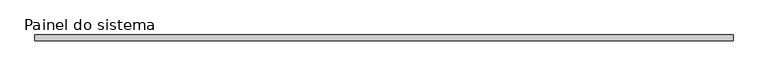
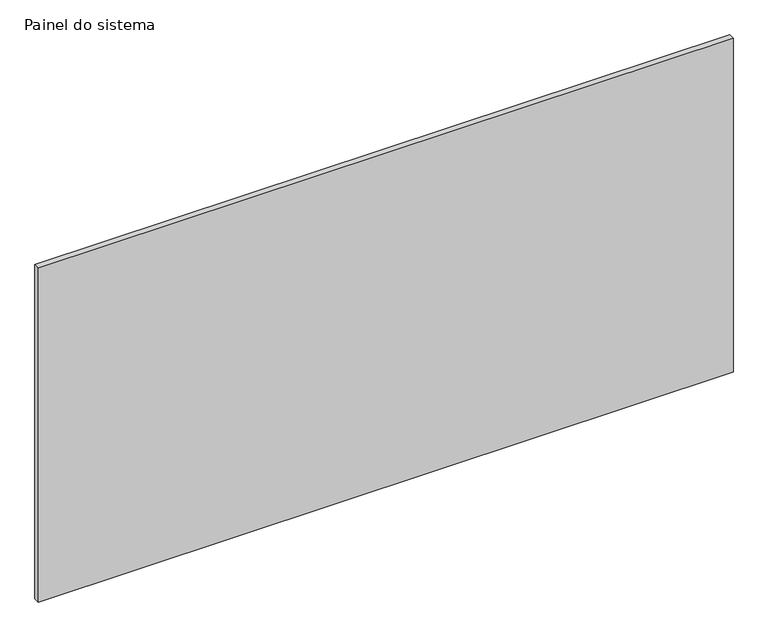
"""IFC4 building model written with IfcOpenShell, lengths in millimetres: plate geometry, Painel do sistema : Envidraçado."""

from ifc_helpers import new_model, si_unit, origin, origin_with_axes, place, context, project, spatial, polyline, outline, extrude, source, transform, mapped, element, save


def painel_do_sistema_85ccde5d(model_context):
    return source(origin(), model_context, "Body", "SweptSolid", [
        extrude(outline(polyline([(1475.0, -49.5), (-1475.0, -49.5), (-1475.0, -24.5), (1475.0, -24.5), (1475.0, -49.5)])), origin_with_axes(), (0.0, 0.0, 1.0), 1500.0),
    ])


if __name__ == "__main__":
    model = new_model("IFC4")
    model_context = context("Model", 3, world=origin())
    ifc_project = project(units=[si_unit("LENGTHUNIT", "METRE", prefix="MILLI")], contexts=[model_context])
    site = spatial("IfcSite", under=ifc_project)
    building = spatial("IfcBuilding", under=site)
    placement = place(None, origin())
    painel_do_sistema_shape = painel_do_sistema_85ccde5d(model_context)
    element("IfcPlate", 1, ObjectType="Painel do sistema : Envidraçado", at=placement, inside=building, context=model_context, shape_type="MappedRepresentation", body=[
        mapped(painel_do_sistema_shape, transform((0.0, 0.0, 0.0), x_axis=(1.0, 0.0, 0.0), y_axis=(0.0, 1.0, 0.0), z_axis=(0.0, 0.0, 1.0))),
    ])
    save(model, "model.ifc")

# Revit data of these elements
# Type "Painel do sistema : Envidraçado"
#   Construction Type Id = "GSP4R"
#   Analytic Construction = "Vidraça única Pilkington 1/8 pol"
#   Visual Light Transmittance = 0.9
#   Solar Heat Gain Coefficient = 0.86
#   Heat Transfer Coefficient (U) = 6.7069 W/(m²·K)
# Element 1 (IfcPlate, "Painel do sistema : Envidraçado")
#   Materials on its faces: "Vidro"
# Materials
#   "Vidro": class "Vidro", colour RGB 0 128 192, transparency 0.9, Description = "Vidro de sílica", Cost = 0
